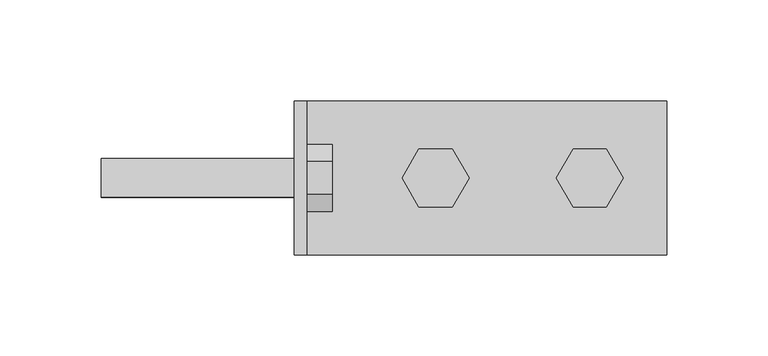
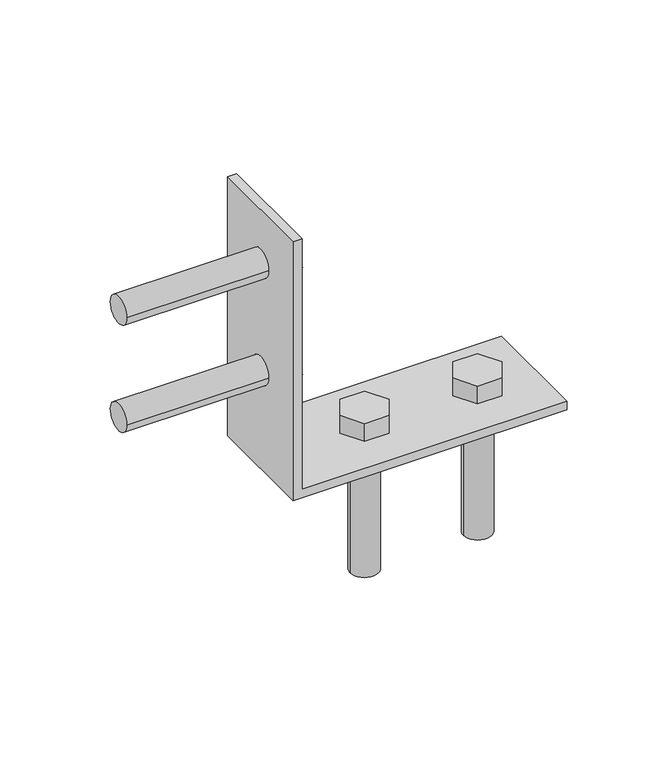
"""IFC4 building model written with IfcOpenShell, lengths in millimetres: fastener geometry, SIMPSON - HLPC/HLGPC Heavy Angles and Gussets : SIMPSON -HL73 - 3 X 7.25 - .75 Bolt - HDG."""

from ifc_helpers import new_model, si_unit, point, frame, frame_2d, origin, place, context, project, spatial, polyline, circle_curve, trimmed, segment, composite_curve, outline, extrude, source, transform, mapped, element, save
from ifc_brep_helpers import plane_surface, revolved_surface, advanced_brep


def fastener_5e5bee1c(model_context):
    return source(origin(), model_context, "Body", "SolidModel", [
        extrude(outline(composite_curve([segment(trimmed(circle_curve(frame_2d((0.0, 69.85)), 9.525), [point((9.525, 69.85))], [point((-9.525, 69.85))], False, "CARTESIAN"), True, "CONTINUOUS"), segment(trimmed(circle_curve(frame_2d((0.0, 69.85)), 9.525), [point((-9.525, 69.85))], [point((9.525, 69.85))], False, "CARTESIAN"), True, "CONTINUOUS")], self_intersect=False)), frame((-95.5476562, 0.0, 0.0), z_axis=(1.0, 0.0, 0.0), x_axis=(0.0, 1.0, 0.0)), (0.0, 0.0, 1.0), 101.6),
        extrude(outline(polyline([(16.4977839, 69.85), (8.248892, 55.5625), (-8.248892, 55.5625), (-16.4977839, 69.85), (-8.248892, 84.1375), (8.248892, 84.1375), (16.4977839, 69.85)])), frame((6.0523438, 0.0, 0.0), z_axis=(1.0, 0.0, 0.0), x_axis=(0.0, 1.0, 0.0)), (0.0, 0.0, 1.0), 12.7),
        extrude(outline(composite_curve([segment(trimmed(circle_curve(frame_2d((0.0, 146.05)), 9.525), [point((9.525, 146.05))], [point((-9.525, 146.05))], False, "CARTESIAN"), True, "CONTINUOUS"), segment(trimmed(circle_curve(frame_2d((0.0, 146.05)), 9.525), [point((-9.525, 146.05))], [point((9.525, 146.05))], False, "CARTESIAN"), True, "CONTINUOUS")], self_intersect=False)), frame((-95.5476562, 0.0, 0.0), z_axis=(1.0, 0.0, 0.0), x_axis=(0.0, 1.0, 0.0)), (0.0, 0.0, 1.0), 101.6),
        extrude(outline(polyline([(16.4977839, 146.05), (8.248892, 131.7625), (-8.248892, 131.7625), (-16.4977839, 146.05), (-8.248892, 160.3375), (8.248892, 160.3375), (16.4977839, 146.05)])), frame((6.0523438, 0.0, 0.0), z_axis=(1.0, 0.0, 0.0), x_axis=(0.0, 1.0, 0.0)), (0.0, 0.0, 1.0), 12.7),
        extrude(outline(composite_curve([segment(trimmed(circle_curve(frame_2d((146.05, 0.0)), 9.525), [point((136.525, 0.0))], [point((155.575, 0.0))], False, "CARTESIAN"), True, "CONTINUOUS"), segment(trimmed(circle_curve(frame_2d((146.05, 0.0)), 9.525), [point((155.575, 0.0))], [point((136.525, 0.0))], False, "CARTESIAN"), True, "CONTINUOUS")], self_intersect=False)), frame((0.0, 0.0, -95.5476563), z_axis=(0.0, 0.0, 1.0), x_axis=(1.0, 0.0, 0.0)), (0.0, 0.0, 1.0), 101.6),
        extrude(outline(polyline([(129.5522161, 0.0), (137.801108, 14.2875), (154.298892, 14.2875), (162.5477839, 0.0), (154.298892, -14.2875), (137.801108, -14.2875), (129.5522161, 0.0)])), frame((0.0, 0.0, 6.0523437), z_axis=(0.0, 0.0, 1.0), x_axis=(1.0, 0.0, 0.0)), (0.0, 0.0, 1.0), 12.7),
        extrude(outline(composite_curve([segment(trimmed(circle_curve(frame_2d((69.85, 0.0)), 9.525), [point((60.325, 0.0))], [point((79.375, 0.0))], False, "CARTESIAN"), True, "CONTINUOUS"), segment(trimmed(circle_curve(frame_2d((69.85, 0.0)), 9.525), [point((79.375, 0.0))], [point((60.325, 0.0))], False, "CARTESIAN"), True, "CONTINUOUS")], self_intersect=False)), frame((0.0, 0.0, -95.5476563), z_axis=(0.0, 0.0, 1.0), x_axis=(1.0, 0.0, 0.0)), (0.0, 0.0, 1.0), 101.6),
        extrude(outline(polyline([(53.3522161, 0.0), (61.601108, 14.2875), (78.098892, 14.2875), (86.3477839, 0.0), (78.098892, -14.2875), (61.601108, -14.2875), (53.3522161, 0.0)])), frame((0.0, 0.0, 6.0523437), z_axis=(0.0, 0.0, 1.0), x_axis=(1.0, 0.0, 0.0)), (0.0, 0.0, 1.0), 12.7),
        advanced_brep(
        [(6.0523438, -38.1, 184.15), (6.0523438, -38.1, 6.0523437), (6.0523438, 38.1, 6.0523437), (6.0523438, 38.1, 184.15), (6.0523438, -9.525, 69.85), (6.0523438, 9.525, 69.85), (6.0523438, -9.525, 146.05), (6.0523438, 9.525, 146.05), (0.0, 38.1, 184.15), (0.0, 38.1, 0.0), (0.0, -38.1, 0.0), (0.0, -38.1, 184.15), (0.0, 9.525, 69.85), (0.0, -9.525, 69.85), (0.0, 9.525, 146.05), (0.0, -9.525, 146.05), (184.15, 38.1, 6.0523437), (184.15, 38.1, 0.0), (184.15, -38.1, 0.0), (184.15, -38.1, 6.0523437), (79.375, 0.0, 6.0523437), (60.325, 0.0, 6.0523437), (155.575, 0.0, 6.0523437), (136.525, 0.0, 6.0523437), (60.325, 0.0, 0.0), (79.375, 0.0, 0.0), (136.525, 0.0, 0.0), (155.575, 0.0, 0.0)],
        [
            (0, 1),
            (1, 2),
            (2, 3),
            (3, 0),
            (4, 5, circle_curve(frame((6.0523438, 0.0, 69.85), z_axis=(-1.0, 0.0, 0.0), x_axis=(0.0, -1.0, 0.0)), 9.525)),
            (5, 4, circle_curve(frame((6.0523438, 0.0, 69.85), z_axis=(-1.0, 0.0, 0.0), x_axis=(0.0, -1.0, 0.0)), 9.525)),
            (6, 7, circle_curve(frame((6.0523438, 0.0, 146.05), z_axis=(-1.0, 0.0, 0.0), x_axis=(0.0, -1.0, 0.0)), 9.525)),
            (7, 6, circle_curve(frame((6.0523438, 0.0, 146.05), z_axis=(-1.0, 0.0, 0.0), x_axis=(0.0, -1.0, 0.0)), 9.525)),
            (8, 9),
            (9, 10),
            (10, 11),
            (11, 8),
            (12, 13, circle_curve(frame((0.0, 0.0, 69.85), z_axis=(1.0, 0.0, 0.0), x_axis=(0.0, -1.0, 0.0)), 9.525)),
            (13, 12, circle_curve(frame((0.0, 0.0, 69.85), z_axis=(1.0, 0.0, 0.0), x_axis=(0.0, -1.0, 0.0)), 9.525)),
            (14, 15, circle_curve(frame((0.0, 0.0, 146.05), z_axis=(1.0, 0.0, 0.0), x_axis=(0.0, -1.0, 0.0)), 9.525)),
            (15, 14, circle_curve(frame((0.0, 0.0, 146.05), z_axis=(1.0, 0.0, 0.0), x_axis=(0.0, -1.0, 0.0)), 9.525)),
            (3, 8),
            (11, 0),
            (2, 16),
            (16, 17),
            (17, 9),
            (10, 18),
            (18, 19),
            (19, 1),
            (19, 16),
            (20, 21, circle_curve(frame((69.85, 0.0, 6.0523437), z_axis=(0.0, 0.0, -1.0), x_axis=(1.0, 0.0, 0.0)), 9.525)),
            (21, 20, circle_curve(frame((69.85, 0.0, 6.0523437), z_axis=(0.0, 0.0, -1.0), x_axis=(1.0, 0.0, 0.0)), 9.525)),
            (22, 23, circle_curve(frame((146.05, 0.0, 6.0523437), z_axis=(0.0, 0.0, -1.0), x_axis=(1.0, 0.0, 0.0)), 9.525)),
            (23, 22, circle_curve(frame((146.05, 0.0, 6.0523437), z_axis=(0.0, 0.0, -1.0), x_axis=(1.0, 0.0, 0.0)), 9.525)),
            (17, 18),
            (24, 25, circle_curve(frame((69.85, 0.0, 0.0), z_axis=(0.0, 0.0, 1.0), x_axis=(1.0, 0.0, 0.0)), 9.525)),
            (25, 24, circle_curve(frame((69.85, 0.0, 0.0), z_axis=(0.0, 0.0, 1.0), x_axis=(1.0, 0.0, 0.0)), 9.525)),
            (26, 27, circle_curve(frame((146.05, 0.0, 0.0), z_axis=(0.0, 0.0, 1.0), x_axis=(1.0, 0.0, 0.0)), 9.525)),
            (27, 26, circle_curve(frame((146.05, 0.0, 0.0), z_axis=(0.0, 0.0, 1.0), x_axis=(1.0, 0.0, 0.0)), 9.525)),
            (21, 24),
            (25, 20),
            (23, 26),
            (27, 22),
            (5, 12),
            (13, 4),
            (7, 14),
            (15, 6),
        ],
        [
            plane_surface(frame((6.0523438, 38.1, 184.15), z_axis=(1.0, 0.0, 0.0), x_axis=(0.0, 1.0, 0.0))),
            plane_surface(frame((0.0, 38.1, 184.15), z_axis=(-1.0, 0.0, 0.0), x_axis=(0.0, -1.0, 0.0))),
            plane_surface(frame((6.0523438, -38.1, 184.15), z_axis=(0.0, 0.0, 1.0), x_axis=(-1.0, 0.0, 0.0))),
            plane_surface(frame((6.0523438, 38.1, 184.15), z_axis=(0.0, 1.0, 0.0), x_axis=(-1.0, 0.0, 0.0))),
            plane_surface(frame((6.0523438, -38.1, 6.0523437), z_axis=(0.0, -1.0, 0.0), x_axis=(-1.0, 0.0, 0.0))),
            plane_surface(frame((0.0, -38.1, 6.0523437), z_axis=(0.0, 0.0, 1.0), x_axis=(-1.0, 0.0, 0.0))),
            plane_surface(frame((0.0, -38.1, 0.0), z_axis=(0.0, 0.0, -1.0), x_axis=(1.0, 0.0, 0.0))),
            plane_surface(frame((184.15, 38.1, 6.0523437), z_axis=(1.0, 0.0, 0.0), x_axis=(0.0, 0.0, -1.0))),
            revolved_surface(polyline([(79.375, 0.0, 6.0523437), (79.375, 0.0, 0.0)]), (69.85, 0.0, 0.0), (0.0, 0.0, 1.0)),
            revolved_surface(polyline([(155.57500000000002, 0.0, 6.0523437), (155.57500000000002, 0.0, 0.0)]), (146.05, 0.0, 0.0), (0.0, 0.0, 1.0)),
            revolved_surface(polyline([(6.0523438, -9.525, 69.85), (0.0, -9.525, 69.85)]), (0.0, 0.0, 69.85), (1.0, 0.0, 0.0)),
            revolved_surface(polyline([(6.0523438, -9.525, 146.05), (0.0, -9.525, 146.05)]), (0.0, 0.0, 146.05), (1.0, 0.0, 0.0)),
        ],
        [
            (0, [[1, 2, 3, 4], [5, 6], [7, 8]]),
            (1, [[9, 10, 11, 12], [13, 14], [15, 16]]),
            (2, [[17, -12, 18, -4]]),
            (3, [[19, 20, 21, -9, -17, -3]]),
            (4, [[-18, -11, 22, 23, 24, -1]]),
            (5, [[-19, -2, -24, 25], [26, 27], [28, 29]]),
            (6, [[-22, -10, -21, 30], [31, 32], [33, 34]]),
            (7, [[-23, -30, -20, -25]]),
            (8, [[-27, 35, -32, 36]]),
            (8, [[-31, -35, -26, -36]]),
            (9, [[-29, 37, -34, 38]]),
            (9, [[-33, -37, -28, -38]]),
            (10, [[-6, 39, -14, 40]]),
            (10, [[-13, -39, -5, -40]]),
            (11, [[-8, 41, -16, 42]]),
            (11, [[-15, -41, -7, -42]]),
        ],
    ),
    ])


if __name__ == "__main__":
    model = new_model("IFC4")
    model_context = context("Model", 3, world=origin())
    ifc_project = project(units=[si_unit("LENGTHUNIT", "METRE", prefix="MILLI")], contexts=[model_context])
    site = spatial("IfcSite", under=ifc_project)
    building = spatial("IfcBuilding", under=site)
    placement = place(None, origin())
    fastener_shape = fastener_5e5bee1c(model_context)
    element("IfcFastener", 1, ObjectType="SIMPSON - HLPC/HLGPC Heavy Angles and Gussets : SIMPSON -HL73 - 3 X 7.25 - .75 Bolt - HDG", at=placement, inside=building, context=model_context, shape_type="MappedRepresentation", body=[
        mapped(fastener_shape, transform((0.0, 0.0, 0.0), x_axis=(1.0, 0.0, 0.0), y_axis=(0.0, 1.0, 0.0), z_axis=(0.0, 0.0, 1.0))),
    ])
    save(model, "model.ifc")

# Revit data of these elements
# Type "SIMPSON - HLPC/HLGPC Heavy Angles and Gussets : SIMPSON -HL73 - 3 X 7.25 - .75 Bolt - HDG"
#   URL = "https://www.strongtie.com/classiccollection_architecturalproductsgroup/hlpc-hlgpc_productgroup_wcc/p/hlpc.hlgpc"
#   L = 0' - 3"
#   Hole Radius = 0' - 0 3/8"
#   D4 = 0' - 3"
#   D2 = 0' - 5"
#   D1 = 0' - 1 1/2"
#   D3 = 0' - 2 3/4"
#   Ga. = 0' - 0 61/256"
#   W1 & W2 = 0' - 7 1/4"
#   Default Elevation = 4' - 0"
#   Bolt Visibility - 3B = no
#   Bolt Visibility - 3A = no
#   Bolt Visibility - 2B = no
#   Bolt Visibility - 2A = no
#   Bolt Visibility - 1B = yes
#   Bolt Visibility - 1A = yes
#   Bolt Visibility = yes
#   Bolt Size = element 1298415
# Element 1 (IfcFastener, "SIMPSON - HLPC/HLGPC Heavy Angles and Gussets : SIMPSON -HL73 - 3 X 7.25 - .75 Bolt - HDG")
#   Materials on its faces: "1\" GALV. LAG BOLT (LENGTH = 1/2\" SHY OF GLULAM DEPTH) -  (GALV. THRU BOLT IF PLATE ON OPP. SIDE OF STRUCT MEMBER)"
# Materials
#   "1\" GALV. LAG BOLT (LENGTH = 1/2\" SHY OF GLULAM DEPTH) -  (GALV. THRU BOLT IF PLATE ON OPP. SIDE OF STRUCT MEMBER)": class "Generic", colour RGB 120 120 120, transparency 0, Cost = 0
